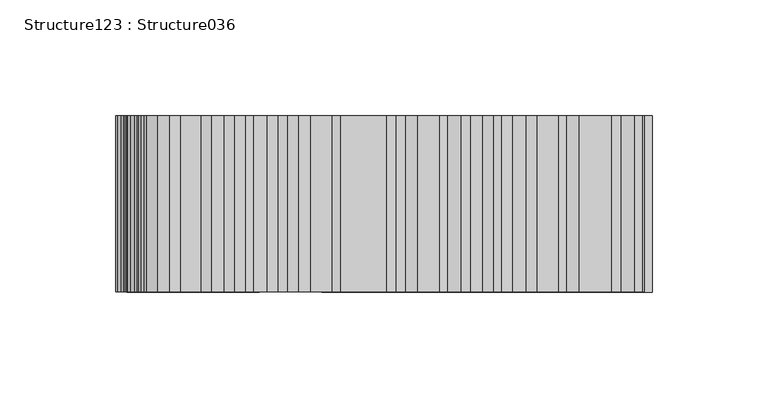
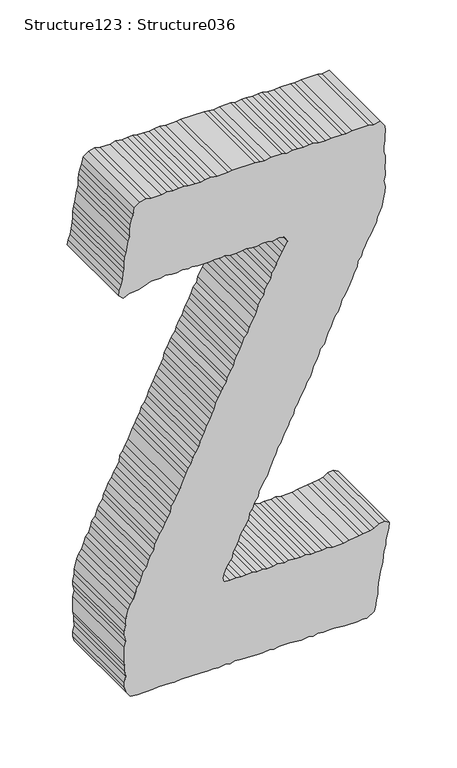
"""IFC4 building model written with IfcOpenShell, lengths in millimetres: proxy geometry, Structure123 : Structure036."""

from ifc_helpers import new_model, si_unit, frame, origin, place, context, project, spatial, polyline, outline, extrude, source, transform, mapped, element, save


def structure123_structure036_cbbf3cad(model_context):
    return source(origin(), model_context, "Body", "SweptSolid", [
        extrude(outline(polyline([(3631.3410106, -45680.1783371), (3633.6821286, -45684.2781015), (3633.0980525, -45688.9715697), (3630.7392839, -45693.0729388), (3629.5984101, -45696.5902318), (3628.998288, -45702.4486428), (3628.4158166, -45705.9739589), (3627.2396415, -45714.7479363), (3626.0554434, -45719.4414045), (3626.0554434, -45728.8090855), (3627.2396415, -45733.4993444), (3626.0554434, -45737.6007135), (3626.6571701, -45743.4687522), (3626.0554434, -45746.9860452), (3627.2396415, -45751.6602581), (3626.6571701, -45756.3521217), (3626.6571701, -45761.0455898), (3627.2396415, -45766.3119018), (3626.0554434, -45769.8372179), (3627.2396415, -45775.6876058), (3626.6571701, -45779.796998), (3626.0554434, -45785.0633099), (3626.6571701, -45788.5709753), (3626.0554434, -45793.2644435), (3627.2396415, -45797.3626034), (3626.6571701, -45802.646566), (3626.6571701, -45807.3320111), (3627.2396415, -45811.4237526), (3626.6571701, -45816.6980875), (3627.2396415, -45821.9820501), (3630.7392839, -45823.1502022), (3634.2822506, -45821.9820501), (3639.5405396, -45820.2153806), (3642.4833842, -45818.4663617), (3647.1575971, -45814.9410456), (3651.2589662, -45814.3649926), (3655.3587307, -45812.0158516), (3660.0682449, -45809.6747337), (3665.3265338, -45807.9160871), (3672.9435914, -45802.646566), (3677.0449604, -45800.881501), (3681.7271964, -45800.2990296), (3685.8285655, -45797.3626034), (3689.9540036, -45796.1880329), (3694.6298211, -45792.6803675), (3698.1294635, -45792.0962914), (3706.3289925, -45787.9965269), (3710.4560353, -45785.0633099), (3716.2887726, -45782.7205873), (3720.4158154, -45780.9715684), (3723.3313817, -45779.796998), (3727.4311462, -45777.4462524), (3732.7167134, -45775.6876058), (3736.2163558, -45773.3448833), (3740.3161203, -45771.5862368), (3744.9999608, -45769.2451188), (3749.117376, -45766.8959778), (3753.2171405, -45765.7278257), (3758.485057, -45762.2201603), (3762.5848215, -45761.6280613), (3766.684586, -45758.6948442), (3771.3860772, -45756.9442207), (3775.4874463, -45754.6031028), (3779.5872107, -45752.2507526), (3783.0868532, -45751.0777867), (3787.2042683, -45748.1413605), (3791.8865042, -45746.3923416), (3795.4037973, -45745.2177711), (3800.6717138, -45742.2925771), (3804.7730829, -45740.5243029), (3809.4729695, -45739.3673831), (3812.3901405, -45735.8516946), (3821.1737455, -45732.90885), (3825.849563, -45730.5757551), (3830.5574726, -45728.8090855), (3834.6588416, -45727.058462), (3838.1761347, -45724.133268), (3843.432819, -45721.7825224), (3847.5598618, -45721.192028), (3850.4754282, -45718.2652294), (3855.7353217, -45715.9225068), (3859.2606378, -45714.1638603), (3863.9332461, -45711.8243469), (3867.4601667, -45710.6481718), (3872.745734, -45707.7229778), (3877.4456205, -45707.1308788), (3880.9452629, -45704.2072894), (3885.6210804, -45703.0295097), (3889.7208449, -45700.6883917), (3893.822214, -45698.9297452), (3897.9476522, -45696.0061558), (3901.44569, -45694.2475093), (3906.7328618, -45691.3126876), (3911.4054701, -45690.7398438), (3919.6066036, -45686.6304517), (3928.4158823, -45684.8718052), (3931.9058971, -45684.2781015), (3937.1930689, -45683.6940255), (3942.4770315, -45684.8718052), (3947.1496398, -45683.6940255), (3950.0940891, -45683.6940255), (3954.7506513, -45684.2781015), (3960.0602876, -45683.6940255), (3964.7361051, -45683.6940255), (3968.8198235, -45684.8718052), (3974.1214368, -45684.8718052), (3978.8036727, -45684.2781015), (3982.8793681, -45684.2781015), (3988.1633307, -45683.6940255), (3992.2614906, -45684.2781015), (3997.5486624, -45687.7953946), (3996.390138, -45693.6634332), (3997.5486624, -45697.7648023), (3997.5486624, -45711.8243469), (3996.390138, -45717.1002865), (3996.9645864, -45720.6159749), (3996.9645864, -45729.983656), (3996.390138, -45734.6739149), (3996.390138, -45740.5243029), (3997.5486624, -45745.2177711), (3997.5486624, -45748.7350641), (3996.9645864, -45753.4285323), (3997.5486624, -45758.6948442), (3997.5486624, -45762.7946087), (3996.390138, -45768.6610428), (3997.5486624, -45772.1799404), (3997.5486624, -45781.5460169), (3996.390138, -45786.8219564), (3996.9645864, -45790.9217209), (3997.5486624, -45795.0327176), (3997.5486624, -45814.9410456), (3996.9645864, -45818.4663617), (3996.9645864, -45827.8324381), (3997.5486624, -45833.1083777), (3996.9645864, -45837.7922182), (3996.390138, -45841.8935873), (3996.390138, -45846.5838463), (3996.9645864, -45852.4342343), (3997.5486624, -45855.9595503), (3997.5486624, -45860.6449955), (3996.9645864, -45865.3352544), (3997.5486624, -45870.6127986), (3996.390138, -45875.2870115), (3996.390138, -45884.0882672), (3997.5486624, -45888.7721077), (3996.390138, -45894.0384196), (3992.8375436, -45898.7318878), (3987.0048063, -45899.9064583), (3983.4794902, -45901.0746103), (3978.8036727, -45902.2491808), (3974.1214368, -45902.8332569), (3968.8198235, -45902.8332569), (3964.7361051, -45904.0062228), (3954.7506513, -45905.7568463), (3951.2606365, -45906.9314168), (3946.5511223, -45907.5235158), (3940.718385, -45907.5235158), (3937.1930689, -45908.1172195), (3931.3346579, -45908.6916679), (3926.6492128, -45909.8662384), (3922.5494483, -45911.6248849), (3917.8479571, -45912.216984), (3914.3499193, -45908.1172195), (3916.6653636, -45903.4237513), (3917.2735087, -45899.3127546), (3917.8479571, -45894.6305187), (3919.0321552, -45890.5211266), (3921.3748778, -45884.6707386), (3921.3748778, -45876.469605), (3922.5494483, -45872.3634221), (3921.3748778, -45866.5130341), (3921.3748778, -45862.411665), (3922.5494483, -45857.7181969), (3921.3748778, -45852.4342343), (3922.5494483, -45849.5106449), (3921.3748778, -45844.2443329), (3921.3748778, -45834.2765298), (3921.9733953, -45830.7672598), (3921.9733953, -45824.9088487), (3922.5494483, -45820.8074797), (3921.3748778, -45816.6980875), (3921.3748778, -45811.4237526), (3921.9733953, -45806.7479351), (3922.5494483, -45803.230642), (3921.3748778, -45797.956307), (3921.3748778, -45793.8469149), (3922.5494483, -45789.164679), (3922.5494483, -45785.0633099), (3921.3748778, -45780.3794694), (3922.5494483, -45775.1035298), (3921.3748778, -45770.4132709), (3916.6653636, -45767.4864723), (3912.5896682, -45769.8372179), (3909.0627475, -45772.1799404), (3904.9645876, -45773.9289593), (3900.2887701, -45776.8621763), (3895.5888836, -45778.6111952), (3892.6636896, -45780.9715684), (3887.9621984, -45781.5460169), (3883.8881076, -45784.4792339), (3879.7610648, -45786.8219564), (3875.0772243, -45787.4140555), (3871.5599312, -45790.3392495), (3867.4601667, -45792.6803675), (3862.2018778, -45793.8469149), (3857.5019912, -45796.1880329), (3850.4754282, -45800.2990296), (3845.1914656, -45801.4639725), (3842.2758992, -45804.3987941), (3837.6000817, -45806.1574406), (3833.4730389, -45807.9160871), (3828.2163546, -45810.8493042), (3824.1149855, -45812.5983231), (3820.015221, -45813.7744982), (3816.4883003, -45816.1140115), (3811.2043377, -45819.0408101), (3807.714323, -45819.6345138), (3803.0064134, -45823.1502022), (3800.0876378, -45824.3167497), (3795.4037973, -45826.6578676), (3791.3056374, -45829.0102178), (3786.6298199, -45830.1751607), (3783.0868532, -45831.9338072), (3778.4046172, -45833.6924538), (3773.7015215, -45836.6272754), (3769.0176809, -45838.3859219), (3765.5019925, -45840.1429638), (3761.418274, -45842.4840818), (3757.3185096, -45843.6602569), (3752.6170184, -45846.0029794), (3749.117376, -45848.9265688), (3743.8414364, -45850.1011393), (3740.9162424, -45852.4342343), (3736.7988273, -45854.2025084), (3732.7167134, -45855.9595503), (3723.9154578, -45860.0512918), (3719.2316172, -45862.411665), (3714.5301261, -45864.74476), (3711.6145597, -45867.0939009), (3706.3289925, -45867.669954), (3702.229228, -45870.0287226), (3698.1294635, -45872.3634221), (3694.029699, -45874.1300917), (3689.9540036, -45877.053681), (3684.6443673, -45879.3964036), (3681.7271964, -45881.1550501), (3677.0449604, -45881.7471492), (3672.3691429, -45885.2644422), (3669.4262983, -45886.4213621), (3663.5598643, -45888.1880316), (3660.6250426, -45891.1148302), (3656.5429288, -45892.2894007), (3651.2589662, -45894.0384196), (3648.3161216, -45896.3891652), (3643.0578326, -45898.1397887), (3638.3563415, -45899.9064583), (3634.2822506, -45902.2491808), (3630.7392839, -45904.0062228), (3622.555801, -45906.3489453), (3617.8559144, -45906.3489453), (3612.0135494, -45907.5235158), (3608.4705827, -45907.5235158), (3602.6298224, -45906.3489453), (3597.9540049, -45907.5235158), (3583.8864372, -45907.5235158), (3580.3691442, -45906.9314168), (3575.6853037, -45906.9314168), (3570.9854171, -45906.3489453), (3565.7094775, -45907.5235158), (3561.6257591, -45907.5235158), (3556.9258725, -45906.3489453), (3551.6675836, -45902.2491808), (3551.0658569, -45896.3891652), (3551.0658569, -45882.904069), (3551.6675836, -45878.2314607), (3551.6675836, -45868.262053), (3551.0658569, -45864.74476), (3551.6675836, -45858.8959766), (3551.6675836, -45841.3095113), (3551.0658569, -45836.6272754), (3551.6675836, -45831.3497312), (3551.0658569, -45826.6578676), (3552.242032, -45820.8074797), (3551.0658569, -45816.6980875), (3552.242032, -45812.5983231), (3551.6675836, -45807.3320111), (3551.6675836, -45798.5403831), (3551.0658569, -45793.8469149), (3551.0658569, -45788.5709753), (3552.242032, -45783.3046634), (3551.0658569, -45779.2048989), (3552.242032, -45774.5114307), (3552.242032, -45765.7278257), (3551.0658569, -45755.7600226), (3552.242032, -45749.9096346), (3551.0658569, -45745.2177711), (3552.242032, -45741.7101056), (3551.6675836, -45737.0166375), (3552.242032, -45731.7503255), (3552.242032, -45727.6409334), (3551.0658569, -45718.2652294), (3551.0658569, -45707.7229778), (3551.6675836, -45703.6232133), (3551.0658569, -45699.5138212), (3555.1848766, -45693.0729388), (3561.025637, -45691.8967637), (3565.1254015, -45691.3126876), (3569.8268927, -45690.1461402), (3573.9266571, -45690.1461402), (3579.7690221, -45689.5540411), (3584.4689087, -45688.9715697), (3589.1527492, -45687.7953946), (3592.6700423, -45687.2225508), (3597.3538828, -45686.0463757), (3602.6298224, -45685.4558812), (3606.7295868, -45684.8718052), (3612.0135494, -45683.1227863), (3616.69739, -45683.1227863), (3621.3732075, -45681.9369836), (3626.0554434, -45680.7624131), (3631.3410106, -45680.1783371)])), frame((0.0, 247945.1599557, 0.0), z_axis=(0.0, 1.0, 0.0), x_axis=(0.0, 0.0, 1.0)), (0.0, 0.0, 1.0), 76.2),
    ])


if __name__ == "__main__":
    model = new_model("IFC4")
    model_context = context("Model", 3, world=origin())
    ifc_project = project(units=[si_unit("LENGTHUNIT", "METRE", prefix="MILLI")], contexts=[model_context])
    site = spatial("IfcSite", under=ifc_project)
    building = spatial("IfcBuilding", under=site)
    placement = place(None, origin())
    structure123_structure036_shape = structure123_structure036_cbbf3cad(model_context)
    element("IfcBuildingElementProxy", 1, Name="Structure123 : Structure036", ObjectType="Structure123 : Structure036", at=placement, inside=building, context=model_context, shape_type="MappedRepresentation", body=[
        mapped(structure123_structure036_shape, transform((0.0, 0.0, 0.0), x_axis=(1.0, 0.0, 0.0), y_axis=(0.0, 1.0, 0.0), z_axis=(0.0, 0.0, 1.0))),
    ])
    save(model, "model.ifc")

# Revit data of these elements
# Type "Structure123 : Structure036"
#   NameOverride = "Structure036"
# Element 1 (IfcBuildingElementProxy, "Structure123 : Structure036")
#   Materials on its faces: "BRUSHED ALUM. LETTERING"
# Materials
#   "BRUSHED ALUM. LETTERING": class "Unassigned", colour RGB 169 181 186, transparency 0, Cost = 0
